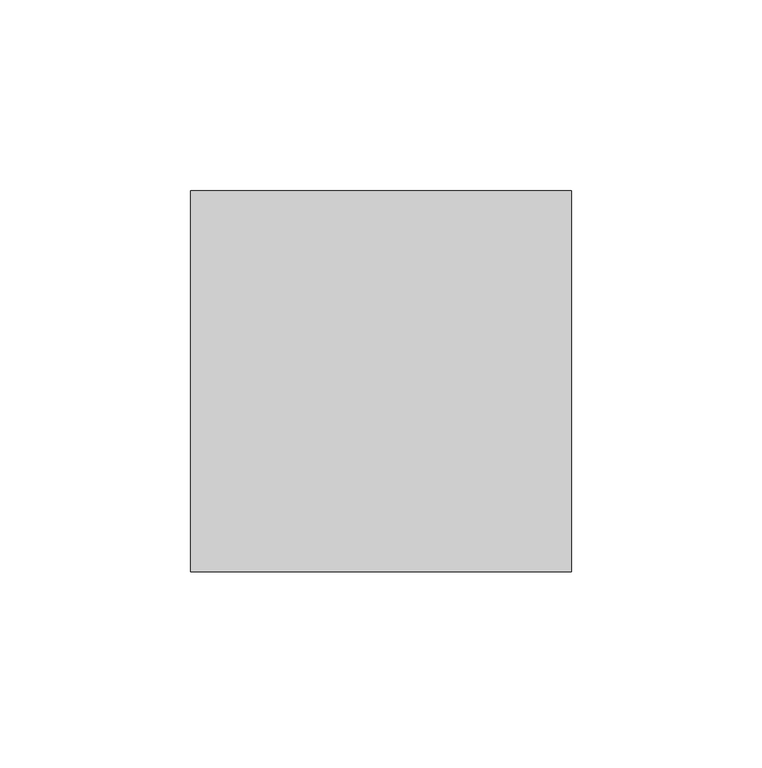
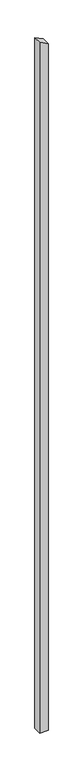
"""IFC4 building model written with IfcOpenShell, lengths in millimetres: column geometry, Holzstütze 158906 : Holzstütze 158906."""

from ifc_helpers import new_model, si_unit, frame, origin, place, context, project, spatial, polyline, outline, extrude, source, transform, mapped, element, save


def column_5ff68a10(model_context):
    return source(origin(), model_context, "Body", "SweptSolid", [
        extrude(outline(polyline([(-500.0, 170467.7593015), (-500.0, 170567.7593015), (8246.2417524, 170567.7593015), (8297.1942973, 170467.7593015), (-500.0, 170467.7593015)])), frame((0.0, 26981.9343946, 0.0), z_axis=(0.0, 1.0, 0.0), x_axis=(0.0, 0.0, 1.0)), (0.0, 0.0, 1.0), 100.0),
    ])


if __name__ == "__main__":
    model = new_model("IFC4")
    model_context = context("Model", 3, world=origin())
    ifc_project = project(units=[si_unit("LENGTHUNIT", "METRE", prefix="MILLI")], contexts=[model_context])
    site = spatial("IfcSite", under=ifc_project)
    building = spatial("IfcBuilding", under=site)
    placement = place(None, origin())
    column_shape = column_5ff68a10(model_context)
    element("IfcColumn", 1, ObjectType="Holzstütze 158906 : Holzstütze 158906", at=placement, inside=building, context=model_context, shape_type="MappedRepresentation", body=[
        mapped(column_shape, transform((0.0, 0.0, 0.0), x_axis=(1.0, 0.0, 0.0), y_axis=(0.0, 1.0, 0.0), z_axis=(0.0, 0.0, 1.0))),
    ])
    save(model, "model.ifc")

# Revit data of these elements
# Type "Holzstütze 158906 : Holzstütze 158906"
#   Abrechnungsart = "m"
#   Allright_Bauteil_ID = "0152St 0000143552"
#   Bezeichnung = "Holzstütze"
#   Codetext = "ST-HOLZ\\"
#   Gewerk = "Zimmer- und Holzbauarbeiten"
#   Material = "Holz"
#   Objektname = "Stütze"
#   NameOverride = "Holzstütze"
#   Reference = "Holzstütze"
#   Status = "NEW"
#   ThermalTransmittance = 0.0000 BTU/(h·ft²·°F)
#   Roll = 0.00°
#   Slope = 0.00°
#   2D Interaktion = yes
#   IsExternal = yes
#   LoadBearing = yes
# Element 1 (IfcColumn, "Holzstütze 158906 : Holzstütze 158906")
#   Materials on its faces: "holzschalung"
# Materials
#   "holzschalung": class "Unassigned", colour RGB 128 128 128, transparency 0
